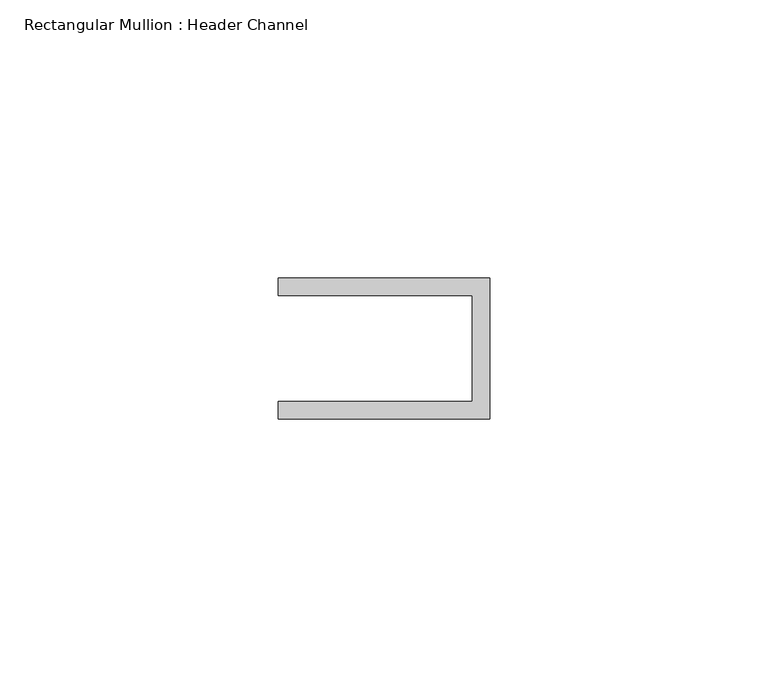
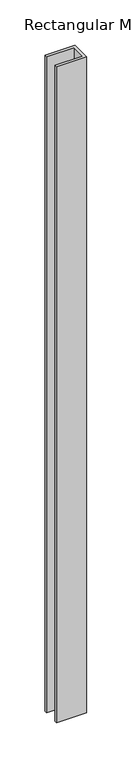
"""IFC4 building model written with IfcOpenShell, lengths in millimetres: member geometry, Rectangular Mullion : Header Channel."""

from ifc_helpers import new_model, si_unit, frame, origin, place, context, project, spatial, polyline, outline, extrude, source, transform, mapped, element, save


def rectangular_mullion_header_channel_aa96db27(model_context):
    return source(origin(), model_context, "Body", "SweptSolid", [
        extrude(outline(polyline([(0.0, -12.7), (-38.1, -12.7), (-38.1, -9.525), (-3.175, -9.525), (-3.175, 9.525), (-38.1, 9.525), (-38.1, 12.7), (0.0, 12.7), (0.0, -12.7)])), frame((0.0, 0.0, -883.3407348), z_axis=(0.0, 0.0, 1.0), x_axis=(1.0, 0.0, 0.0)), (0.0, 0.0, 1.0), 883.3407348),
    ])


if __name__ == "__main__":
    model = new_model("IFC4")
    model_context = context("Model", 3, world=origin())
    ifc_project = project(units=[si_unit("LENGTHUNIT", "METRE", prefix="MILLI")], contexts=[model_context])
    site = spatial("IfcSite", under=ifc_project)
    building = spatial("IfcBuilding", under=site)
    placement = place(None, origin())
    rectangular_mullion_header_channel_shape = rectangular_mullion_header_channel_aa96db27(model_context)
    element("IfcMember", 1, ObjectType="Rectangular Mullion : Header Channel", at=placement, inside=building, context=model_context, shape_type="MappedRepresentation", body=[
        mapped(rectangular_mullion_header_channel_shape, transform((0.0, 0.0, 0.0), x_axis=(1.0, 0.0, 0.0), y_axis=(0.0, 1.0, 0.0), z_axis=(0.0, 0.0, 1.0))),
    ])
    save(model, "model.ifc")

# Revit data of these elements
# Type "Rectangular Mullion : Header Channel"
#   built-in parameter 1007322 = 0.0833333 (stored number, unit not read)
#   built-in parameter 1007321 = -0.03125 (stored number, unit not read)
#   built-in parameter 1007320 = 0.0416667 (stored number, unit not read)
# Element 1 (IfcMember, "Rectangular Mullion : Header Channel")
#   Materials on its faces: "ALUM"
# Materials
#   "ALUM": class "Generic", colour RGB 157 157 157, transparency 0, Cost = 0
